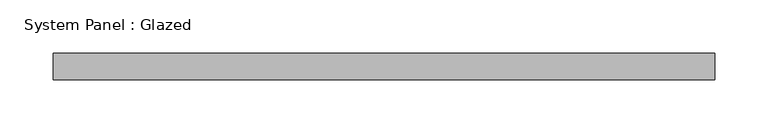
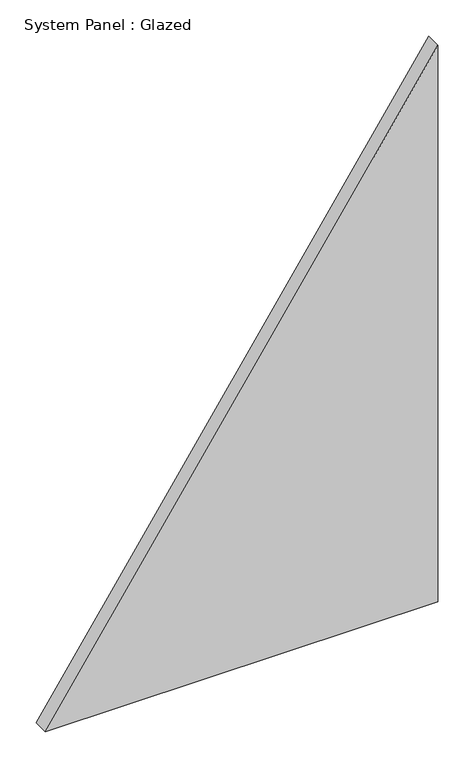
"""IFC4 building model written with IfcOpenShell, lengths in millimetres: plate geometry, System Panel : Glazed."""

import ifcopenshell
import ifcopenshell.guid

model = None  # the IFC model being written
_history = None  # IfcOwnerHistory: only IFC2X3 demands one
_inside = {}  # id of a spatial element -> (the spatial element, [elements in it])
_under = {}  # id of a project, library or spatial element -> (it, [spatial elements below it])
_declared = {}  # id of a project -> (the project, [libraries it declares])
_typed = {}  # id of a type object -> (the type object, [elements of that type])
_made_of = {}  # id of a material, layer set ... -> (it, [elements and type objects made of it])


def new_model(schema):
    """Start an empty IFC model of exactly this schema.

    Asked for "IFC4X3", IfcOpenShell would pick the latest addendum, in which some entities
    have other attributes; the version numbers below select the first issue.
    IFC2X3 requires an IfcOwnerHistory on every rooted entity: one is made here for all.
    """
    global model, _history
    if schema == "IFC4X3":
        model = ifcopenshell.file(schema_version=(4, 3, 0, 0))
    else:
        model = ifcopenshell.file(schema=schema)
    _inside.clear()
    _under.clear()
    _declared.clear()
    _typed.clear()
    _made_of.clear()
    _history = None
    if model.schema == "IFC2X3":
        org = make("IfcOrganization", Name="unknown")
        user = make(
            "IfcPersonAndOrganization",
            ThePerson=make("IfcPerson", FamilyName="unknown"),
            TheOrganization=org,
        )
        app = make(
            "IfcApplication",
            ApplicationDeveloper=org,
            Version="unknown",
            ApplicationFullName="unknown",
            ApplicationIdentifier="unknown",
        )
        _history = make(
            "IfcOwnerHistory",
            OwningUser=user,
            OwningApplication=app,
            ChangeAction="ADDED",
            CreationDate=0,
        )
    return model


def make(cls, **values):
    """One entity of the class cls with the attributes given. An attribute that is None is left unset."""
    return model.create_entity(
        cls, **{name: value for name, value in values.items() if value is not None}
    )


def rooted(cls, **values):
    """An entity with a GlobalId (a new one), such as an element, a storey or a relation."""
    return make(cls, GlobalId=ifcopenshell.guid.new(), OwnerHistory=_history, **values)


def si_unit(unit_type, name, prefix=None):
    """IfcSIUnit, for example si_unit("LENGTHUNIT", "METRE", prefix="MILLI")."""
    return make("IfcSIUnit", UnitType=unit_type, Prefix=prefix, Name=name)


def assignment(units):
    """IfcUnitAssignment: the units of a project."""
    return None if units is None else make("IfcUnitAssignment", Units=units)


def point(xyz):
    """IfcCartesianPoint."""
    return None if xyz is None else make("IfcCartesianPoint", Coordinates=xyz)


def direction(xyz):
    """IfcDirection."""
    return None if xyz is None else make("IfcDirection", DirectionRatios=xyz)


def frame(location, z_axis=None, x_axis=None):
    """IfcAxis2Placement3D, a coordinate frame: its origin and axes. An axis left out is left unset."""
    return make(
        "IfcAxis2Placement3D",
        Location=point(location),
        Axis=direction(z_axis),
        RefDirection=direction(x_axis),
    )


def origin():
    """The frame at (0, 0, 0) with its axes left unset."""
    return frame((0.0, 0.0, 0.0))


def place(relative_to, where):
    """IfcLocalPlacement: puts the frame where relative to a parent placement (None: the world)."""
    return make(
        "IfcLocalPlacement", PlacementRelTo=relative_to, RelativePlacement=where
    )


def context(
    kind, dimensions, precision=None, world=None, true_north=None, identifier=None
):
    """IfcGeometricRepresentationContext, for example the 3D "Model" context."""
    return make(
        "IfcGeometricRepresentationContext",
        ContextIdentifier=identifier,
        ContextType=kind,
        CoordinateSpaceDimension=dimensions,
        Precision=precision,
        WorldCoordinateSystem=world,
        TrueNorth=true_north,
    )


def project(units=None, contexts=None):
    """IfcProject with its units and contexts."""
    return rooted(
        "IfcProject",
        Name="project",
        RepresentationContexts=contexts,
        UnitsInContext=assignment(units),
    )


def spatial(cls, under=None, at=None, **own):
    """A site, building, storey or space (cls), placed at a placement, below another one or the project."""
    s = rooted(cls, ObjectPlacement=at, **own)
    if under is not None:
        _under.setdefault(under.id(), (under, []))[1].append(s)
    return s


def polyline(points):
    """IfcPolyline through the points."""
    return make("IfcPolyline", Points=[point(p) for p in points])


def outline(outer, holes=None, kind="AREA"):
    """IfcArbitraryClosedProfileDef: a profile drawn as a closed curve; with holes, ...WithVoids."""
    if holes is None:
        return make("IfcArbitraryClosedProfileDef", ProfileType=kind, OuterCurve=outer)
    return make(
        "IfcArbitraryProfileDefWithVoids",
        ProfileType=kind,
        OuterCurve=outer,
        InnerCurves=holes,
    )


def extrude(swept, where, along, depth):
    """IfcExtrudedAreaSolid: the profile swept, set in the frame where, extruded along a direction by depth."""
    return make(
        "IfcExtrudedAreaSolid",
        SweptArea=swept,
        Position=where,
        ExtrudedDirection=direction(along),
        Depth=depth,
    )


def shape(context_of_items, identifier, shape_type, items):
    """IfcShapeRepresentation: the items that make up one representation, for example the "Body"."""
    return make(
        "IfcShapeRepresentation",
        ContextOfItems=context_of_items,
        RepresentationIdentifier=identifier,
        RepresentationType=shape_type,
        Items=items,
    )


def source(mapping_origin, context_of_items, identifier, shape_type, items):
    """IfcRepresentationMap: a shape defined once, which mapped items show again and again."""
    return make(
        "IfcRepresentationMap",
        MappingOrigin=mapping_origin,
        MappedRepresentation=shape(context_of_items, identifier, shape_type, items),
    )


def transform(
    local_origin,
    x_axis=None,
    y_axis=None,
    z_axis=None,
    scale=None,
    scale2=None,
    scale3=None,
    uniform=True,
):
    """IfcCartesianTransformationOperator3D, or its non-uniform kind. x_axis, y_axis, z_axis: its Axis1, 2, 3."""
    if uniform:
        return make(
            "IfcCartesianTransformationOperator3D",
            Axis1=direction(x_axis),
            Axis2=direction(y_axis),
            LocalOrigin=point(local_origin),
            Scale=scale,
            Axis3=direction(z_axis),
        )
    return make(
        "IfcCartesianTransformationOperator3DnonUniform",
        Axis1=direction(x_axis),
        Axis2=direction(y_axis),
        LocalOrigin=point(local_origin),
        Scale=scale,
        Axis3=direction(z_axis),
        Scale2=scale2,
        Scale3=scale3,
    )


def mapped(mapping_source, mapping_target):
    """IfcMappedItem: shows the shape of a source again, moved by a transform."""
    return make(
        "IfcMappedItem", MappingSource=mapping_source, MappingTarget=mapping_target
    )


def made_of(thing, what):
    """Note that an element or type object is made of a material, layer set ...; save() writes the relation."""
    if what is not None:
        _made_of.setdefault(what.id(), (what, []))[1].append(thing)
    return thing


def element(
    cls,
    number,
    at=None,
    inside=None,
    cuts=None,
    type_object=None,
    material=None,
    context=None,
    identifier="Body",
    shape_type=None,
    held_by="IfcProductDefinitionShape",
    body=None,
    shapes=None,
    **own,
):
    """One element of the class cls, such as IfcWall. Its Tag is "e" and its number.

    at: its placement. inside: the storey or other place that contains it. cuts: it is an
    opening in that element (IfcRelVoidsElement). A single representation is given by context,
    identifier, shape_type and body (its items); several are given by shapes. held_by: the class
    of the entity that holds the representations. save() writes the other relations.
    """
    e = rooted(cls, Tag="e%d" % number, ObjectPlacement=at, **own)
    if body is not None:
        shapes = [shape(context, identifier, shape_type, body)]
    if shapes is not None:
        e.Representation = make(held_by, Representations=shapes)
    if inside is not None:
        _inside.setdefault(inside.id(), (inside, []))[1].append(e)
    if cuts is not None:
        rooted(
            "IfcRelVoidsElement", RelatingBuildingElement=cuts, RelatedOpeningElement=e
        )
    if type_object is not None:
        _typed.setdefault(type_object.id(), (type_object, []))[1].append(e)
    return made_of(e, material)


def aggregate(whole, parts):
    """IfcRelAggregates: a whole, such as a stair, and the parts it consists of."""
    return rooted("IfcRelAggregates", RelatingObject=whole, RelatedObjects=parts)


def save(model, path):
    """Write the relations noted so far, then the file.

    IfcRelAggregates (storeys below a building ...), IfcRelContainedInSpatialStructure (elements
    in a storey), IfcRelDefinesByType, IfcRelAssociatesMaterial and IfcRelDeclares: one each for
    every whole, place, type object, material and project.
    """
    for whole, parts in _under.values():
        aggregate(whole, parts)
    for where, things in _inside.values():
        rooted(
            "IfcRelContainedInSpatialStructure",
            RelatedElements=things,
            RelatingStructure=where,
        )
    for kind, things in _typed.values():
        rooted("IfcRelDefinesByType", RelatedObjects=things, RelatingType=kind)
    for what, things in _made_of.values():
        rooted("IfcRelAssociatesMaterial", RelatedObjects=things, RelatingMaterial=what)
    for by, libraries in _declared.values():
        rooted("IfcRelDeclares", RelatingContext=by, RelatedDefinitions=libraries)
    model.write(path)


def system_panel_glazed_33dcd8ce(model_context):
    return source(origin(), model_context, "Body", "SweptSolid", [
        extrude(outline(polyline([(0.0, -311.474195), (0.0, 311.474195), (934.2941385, 311.474195), (0.0, -311.474195)])), frame((0.0, 24.5, 0.0), z_axis=(0.0, 1.0, 0.0), x_axis=(0.0, 0.0, 1.0)), (0.0, 0.0, 1.0), 25.0),
    ])


if __name__ == "__main__":
    model = new_model("IFC4")
    model_context = context("Model", 3, world=origin())
    ifc_project = project(units=[si_unit("LENGTHUNIT", "METRE", prefix="MILLI")], contexts=[model_context])
    site = spatial("IfcSite", under=ifc_project)
    building = spatial("IfcBuilding", under=site)
    placement = place(None, origin())
    system_panel_glazed_shape = system_panel_glazed_33dcd8ce(model_context)
    element("IfcPlate", 1, ObjectType="System Panel : Glazed", at=placement, inside=building, context=model_context, shape_type="MappedRepresentation", body=[
        mapped(system_panel_glazed_shape, transform((0.0, 0.0, 0.0), x_axis=(1.0, 0.0, 0.0), y_axis=(0.0, 1.0, 0.0), z_axis=(0.0, 0.0, 1.0))),
    ])
    save(model, "model.ifc")

# Revit data of these elements
# Type "System Panel : Glazed"
#   Keynote = "H11"
#   Construction Type Id = "GSP4R"
#   Analytic Construction = "1/8 in Pilkington single glazing"
#   Visual Light Transmittance = 0.9
#   Solar Heat Gain Coefficient = 0.86
#   Heat Transfer Coefficient (U) = 6.7069 W/(m²·K)
#   Define Thermal Properties by = 1
# Element 1 (IfcPlate, "System Panel : Glazed")
#   Materials on its faces: "Glass"
# Materials
#   "Glass": class "Glass", colour RGB 0 128 192, transparency 0.9, Description = "Soda Lime Glass", Cost = 0
